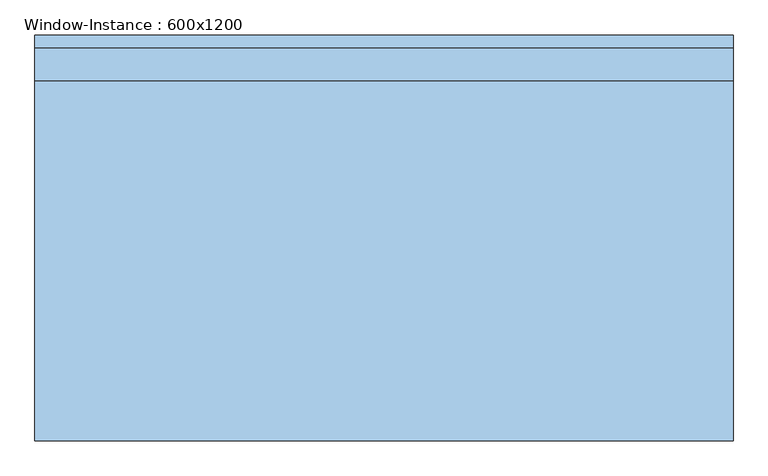
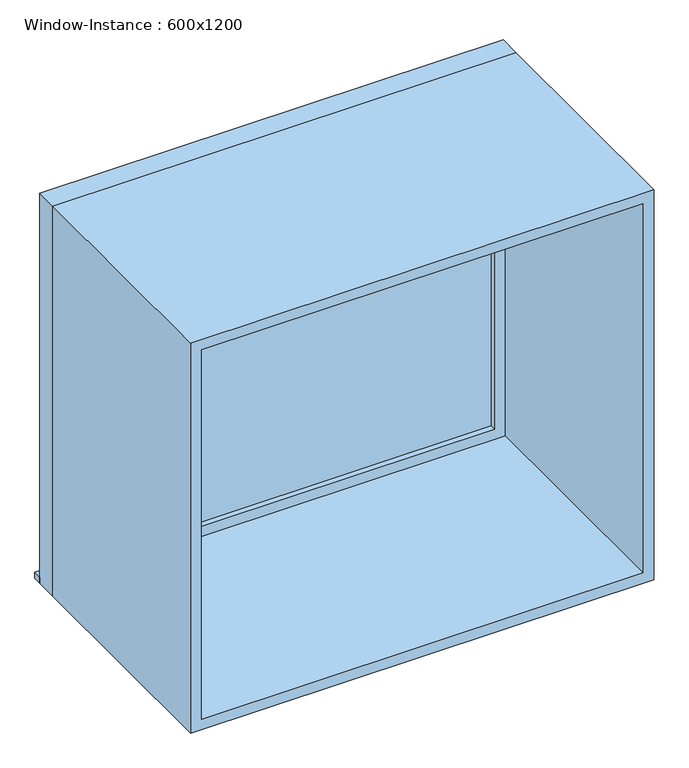
"""IFC4 building model written with IfcOpenShell, lengths in millimetres: window geometry, Window-Instance : 600x1200."""

from ifc_helpers import new_model, si_unit, frame, origin, place, context, project, spatial, polyline, outline, extrude, source, transform, mapped, element, save


def window_instance_600x1200_e847af59(model_context):
    return source(origin(), model_context, "Body", "SweptSolid", [
        extrude(outline(polyline([(-713.1, 405.4), (636.9, 405.4), (636.9, 380.0), (-713.1, 380.0), (-713.1, 405.4)])), frame((0.0, 0.0, 900.0), z_axis=(0.0, 0.0, 1.0), x_axis=(1.0, 0.0, 0.0)), (0.0, 0.0, 1.0), 19.05),
        extrude(outline(polyline([(573.4, 331.425), (-649.6, 331.425), (-649.6, 344.125), (573.4, 344.125), (573.4, 331.425)])), frame((0.0, 0.0, 963.5), z_axis=(0.0, 0.0, 1.0), x_axis=(1.0, 0.0, 0.0)), (0.0, 0.0, 1.0), 1073.0),
        extrude(outline(polyline([(2080.95, -694.05), (919.05, -694.05), (919.05, 617.85), (2080.95, 617.85), (2080.95, -694.05)]), holes=[polyline([(2036.5, -649.6), (2036.5, 573.4), (963.5, 573.4), (963.5, -649.6), (2036.5, -649.6)])]), frame((0.0, 315.55, 0.0), z_axis=(0.0, 1.0, 0.0), x_axis=(0.0, 0.0, 1.0)), (0.0, 0.0, 1.0), 44.45),
        extrude(outline(polyline([(2100.0, -713.1), (900.0, -713.1), (900.0, 636.9), (2100.0, 636.9), (2100.0, -713.1)]), holes=[polyline([(2068.25, -681.35), (2068.25, 605.15), (931.75, 605.15), (931.75, -681.35), (2068.25, -681.35)])]), frame((0.0, -380.0, 0.0), z_axis=(0.0, 1.0, 0.0), x_axis=(0.0, 0.0, 1.0)), (0.0, 0.0, 1.0), 695.55),
        extrude(outline(polyline([(2100.0, 636.9), (2100.0, -713.1), (900.0, -713.1), (900.0, 636.9), (2100.0, 636.9)]), holes=[polyline([(2080.95, 617.85), (919.05, 617.85), (919.05, -694.05), (2080.95, -694.05), (2080.95, 617.85)])]), frame((0.0, 315.55, 0.0), z_axis=(0.0, 1.0, 0.0), x_axis=(0.0, 0.0, 1.0)), (0.0, 0.0, 1.0), 64.45),
    ])


if __name__ == "__main__":
    model = new_model("IFC4")
    model_context = context("Model", 3, world=origin())
    ifc_project = project(units=[si_unit("LENGTHUNIT", "METRE", prefix="MILLI")], contexts=[model_context])
    site = spatial("IfcSite", under=ifc_project)
    building = spatial("IfcBuilding", under=site)
    placement = place(None, origin())
    window_instance_600x1200_shape = window_instance_600x1200_e847af59(model_context)
    element("IfcWindow", 1, ObjectType="Window-Instance : 600x1200", at=placement, inside=building, context=model_context, shape_type="MappedRepresentation", body=[
        mapped(window_instance_600x1200_shape, transform((0.0, 0.0, 0.0), x_axis=(1.0, 0.0, 0.0), y_axis=(0.0, 1.0, 0.0), z_axis=(0.0, 0.0, 1.0))),
    ])
    save(model, "model.ifc")

# Revit data of these elements
# Type "Window-Instance : 600x1200"
#   Type Mark = "7"
#   Construction Type Id = "GSP4R"
#   Assembly Code = "B2020100"
#   Analytic Construction = "1/8 in Pilkington single glazing"
#   Visual Light Transmittance = 0.9
#   Thermal Resistance (R) = 0.149095 (m²·K)/W
#   Solar Heat Gain Coefficient = 0.86
#   Heat Transfer Coefficient (U) = 6.70716 W/(m²·K)
#   Height [instance default] = 1200 mm
#   Default Sill Height = 900 mm
#   Width [instance default] = 600 mm
#   Window Inset = 20 mm
#   Glass Pane Material = WW-EC-GL-Storefront
#   Sash Material = WW-EC-RGB-White
#   Wall Closure = (empty or 0)
# Element 1 (IfcWindow, "Window-Instance : 600x1200")
#   Width = 1350 mm
#   Materials on its faces: "WW-EC-RGB-White", "WW-EC-GL-Storefront"
# Materials
#   "WW-EC-GL-Storefront": class "Glass", colour RGB 236 240 239, transparency 0.85, Description = "Storefront Glass", Cost = 0
#   "WW-EC-RGB-White": class "Generic", colour RGB 255 255 255, transparency 0, Comments = "If region requests off-white, swith asset color to RGB 231-228-220", Description = "Generic Color", Cost = 0
